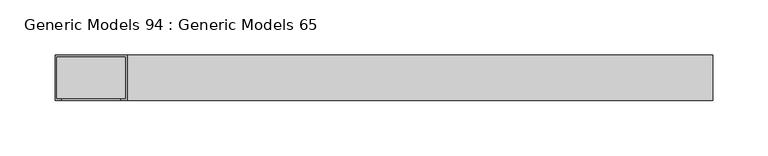
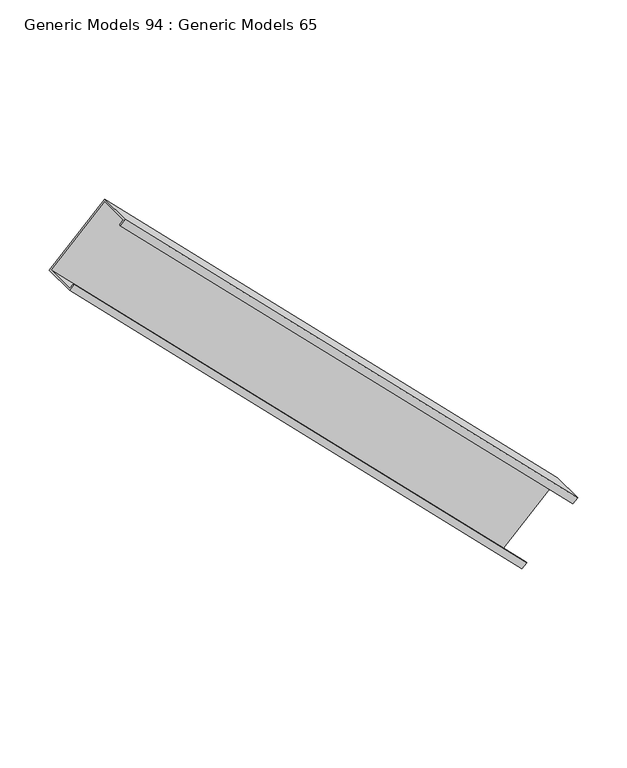
"""IFC4 building model written with IfcOpenShell, lengths in millimetres: proxy geometry, Generic Models 94 : Generic Models 65."""

from ifc_helpers import new_model, si_unit, frame, origin, place, context, project, spatial, polyline, outline, extrude, source, transform, mapped, element, save


def generic_models_94_generic_models_65_e95720d5(model_context):
    return source(origin(), model_context, "Body", "SweptSolid", [
        extrude(outline(polyline([(0.0, -92.075), (0.0, 0.0), (41.275, 0.0), (41.275, -7.9375), (39.6875, -7.9375), (39.6875, -1.5875), (1.5875, -1.5875), (1.5875, -90.4875001), (39.6875, -90.4875001), (39.6875, -84.1375), (41.275, -84.1375), (41.275, -92.075), (0.0, -92.075)])), frame((48147.1360531, 630.2375, 1792.900826), z_axis=(-0.7071067811865384, 0.0, 0.7071067811865568), x_axis=(0.0, -1.0, 0.0)), (0.0, 0.0, 1.0), 749.9641452),
    ])


if __name__ == "__main__":
    model = new_model("IFC4")
    model_context = context("Model", 3, world=origin())
    ifc_project = project(units=[si_unit("LENGTHUNIT", "METRE", prefix="MILLI")], contexts=[model_context])
    site = spatial("IfcSite", under=ifc_project)
    building = spatial("IfcBuilding", under=site)
    placement = place(None, origin())
    generic_models_94_generic_models_65_shape = generic_models_94_generic_models_65_e95720d5(model_context)
    element("IfcBuildingElementProxy", 1, Name="Generic Models 94 : Generic Models 65", ObjectType="Generic Models 94 : Generic Models 65", at=placement, inside=building, context=model_context, shape_type="MappedRepresentation", body=[
        mapped(generic_models_94_generic_models_65_shape, transform((0.0, 0.0, 0.0), x_axis=(1.0, 0.0, 0.0), y_axis=(0.0, 1.0, 0.0), z_axis=(0.0, 0.0, 1.0))),
    ])
    save(model, "model.ifc")

# Revit data of these elements
# Element 1 (IfcBuildingElementProxy, "Generic Models 94 : Generic Models 65")
#   Materials on its faces: "DIAGONAL BRACING AS NECESSARY - ATTACH TO STRUCTURAL DECK"
# Materials
#   "DIAGONAL BRACING AS NECESSARY - ATTACH TO STRUCTURAL DECK": class "Unassigned", colour RGB 210 209 208, transparency 0, Keynote = "M05121300.02", Cost = 0
